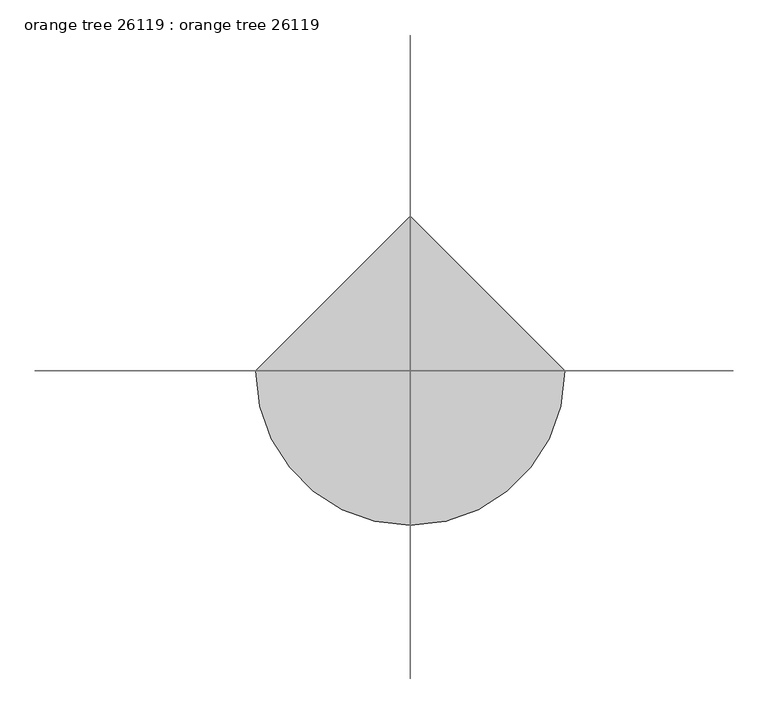
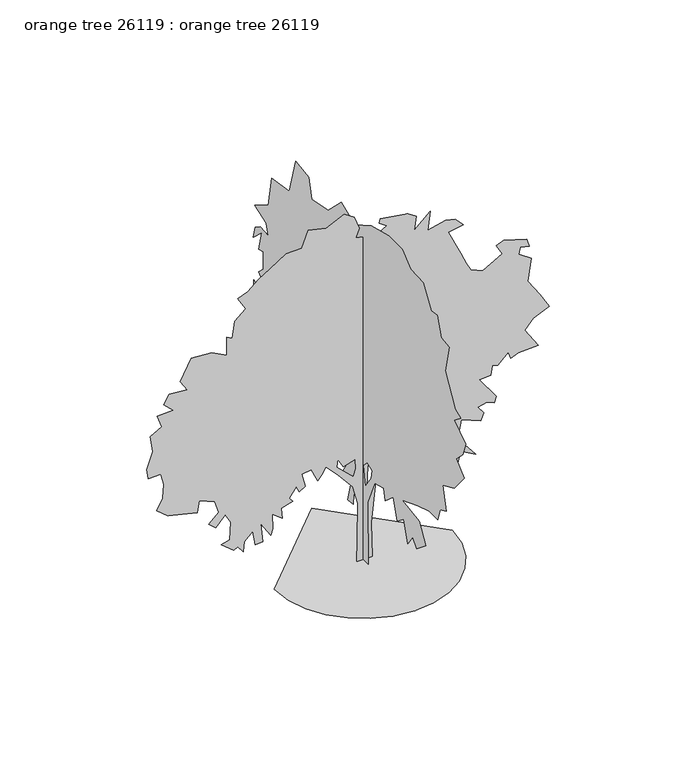
"""IFC4 building model written with IfcOpenShell, lengths in millimetres: proxy geometry, orange tree 26119 : orange tree 26119."""

import ifcopenshell
import ifcopenshell.guid

model = None  # the IFC model being written
_history = None  # IfcOwnerHistory: only IFC2X3 demands one
_inside = {}  # id of a spatial element -> (the spatial element, [elements in it])
_under = {}  # id of a project, library or spatial element -> (it, [spatial elements below it])
_declared = {}  # id of a project -> (the project, [libraries it declares])
_typed = {}  # id of a type object -> (the type object, [elements of that type])
_made_of = {}  # id of a material, layer set ... -> (it, [elements and type objects made of it])


def new_model(schema):
    """Start an empty IFC model of exactly this schema.

    Asked for "IFC4X3", IfcOpenShell would pick the latest addendum, in which some entities
    have other attributes; the version numbers below select the first issue.
    IFC2X3 requires an IfcOwnerHistory on every rooted entity: one is made here for all.
    """
    global model, _history
    if schema == "IFC4X3":
        model = ifcopenshell.file(schema_version=(4, 3, 0, 0))
    else:
        model = ifcopenshell.file(schema=schema)
    _inside.clear()
    _under.clear()
    _declared.clear()
    _typed.clear()
    _made_of.clear()
    _history = None
    if model.schema == "IFC2X3":
        org = make("IfcOrganization", Name="unknown")
        user = make(
            "IfcPersonAndOrganization",
            ThePerson=make("IfcPerson", FamilyName="unknown"),
            TheOrganization=org,
        )
        app = make(
            "IfcApplication",
            ApplicationDeveloper=org,
            Version="unknown",
            ApplicationFullName="unknown",
            ApplicationIdentifier="unknown",
        )
        _history = make(
            "IfcOwnerHistory",
            OwningUser=user,
            OwningApplication=app,
            ChangeAction="ADDED",
            CreationDate=0,
        )
    return model


def make(cls, **values):
    """One entity of the class cls with the attributes given. An attribute that is None is left unset."""
    return model.create_entity(
        cls, **{name: value for name, value in values.items() if value is not None}
    )


def rooted(cls, **values):
    """An entity with a GlobalId (a new one), such as an element, a storey or a relation."""
    return make(cls, GlobalId=ifcopenshell.guid.new(), OwnerHistory=_history, **values)


def si_unit(unit_type, name, prefix=None):
    """IfcSIUnit, for example si_unit("LENGTHUNIT", "METRE", prefix="MILLI")."""
    return make("IfcSIUnit", UnitType=unit_type, Prefix=prefix, Name=name)


def assignment(units):
    """IfcUnitAssignment: the units of a project."""
    return None if units is None else make("IfcUnitAssignment", Units=units)


def point(xyz):
    """IfcCartesianPoint."""
    return None if xyz is None else make("IfcCartesianPoint", Coordinates=xyz)


def direction(xyz):
    """IfcDirection."""
    return None if xyz is None else make("IfcDirection", DirectionRatios=xyz)


def frame(location, z_axis=None, x_axis=None):
    """IfcAxis2Placement3D, a coordinate frame: its origin and axes. An axis left out is left unset."""
    return make(
        "IfcAxis2Placement3D",
        Location=point(location),
        Axis=direction(z_axis),
        RefDirection=direction(x_axis),
    )


def origin():
    """The frame at (0, 0, 0) with its axes left unset."""
    return frame((0.0, 0.0, 0.0))


def place(relative_to, where):
    """IfcLocalPlacement: puts the frame where relative to a parent placement (None: the world)."""
    return make(
        "IfcLocalPlacement", PlacementRelTo=relative_to, RelativePlacement=where
    )


def context(
    kind, dimensions, precision=None, world=None, true_north=None, identifier=None
):
    """IfcGeometricRepresentationContext, for example the 3D "Model" context."""
    return make(
        "IfcGeometricRepresentationContext",
        ContextIdentifier=identifier,
        ContextType=kind,
        CoordinateSpaceDimension=dimensions,
        Precision=precision,
        WorldCoordinateSystem=world,
        TrueNorth=true_north,
    )


def project(units=None, contexts=None):
    """IfcProject with its units and contexts."""
    return rooted(
        "IfcProject",
        Name="project",
        RepresentationContexts=contexts,
        UnitsInContext=assignment(units),
    )


def spatial(cls, under=None, at=None, **own):
    """A site, building, storey or space (cls), placed at a placement, below another one or the project."""
    s = rooted(cls, ObjectPlacement=at, **own)
    if under is not None:
        _under.setdefault(under.id(), (under, []))[1].append(s)
    return s


def point_list(points):
    """IfcCartesianPointList2D or 3D."""
    cls = (
        "IfcCartesianPointList2D" if len(points[0]) == 2 else "IfcCartesianPointList3D"
    )
    return make(cls, CoordList=points)


def triangles(points, corners, closed=None, point_numbers=None):
    """IfcTriangulatedFaceSet: each triangle names its three corners, points numbered from 1."""
    return make(
        "IfcTriangulatedFaceSet",
        Coordinates=point_list(points),
        Closed=closed,
        CoordIndex=corners,
        PnIndex=point_numbers,
    )


def shape(context_of_items, identifier, shape_type, items):
    """IfcShapeRepresentation: the items that make up one representation, for example the "Body"."""
    return make(
        "IfcShapeRepresentation",
        ContextOfItems=context_of_items,
        RepresentationIdentifier=identifier,
        RepresentationType=shape_type,
        Items=items,
    )


def source(mapping_origin, context_of_items, identifier, shape_type, items):
    """IfcRepresentationMap: a shape defined once, which mapped items show again and again."""
    return make(
        "IfcRepresentationMap",
        MappingOrigin=mapping_origin,
        MappedRepresentation=shape(context_of_items, identifier, shape_type, items),
    )


def transform(
    local_origin,
    x_axis=None,
    y_axis=None,
    z_axis=None,
    scale=None,
    scale2=None,
    scale3=None,
    uniform=True,
):
    """IfcCartesianTransformationOperator3D, or its non-uniform kind. x_axis, y_axis, z_axis: its Axis1, 2, 3."""
    if uniform:
        return make(
            "IfcCartesianTransformationOperator3D",
            Axis1=direction(x_axis),
            Axis2=direction(y_axis),
            LocalOrigin=point(local_origin),
            Scale=scale,
            Axis3=direction(z_axis),
        )
    return make(
        "IfcCartesianTransformationOperator3DnonUniform",
        Axis1=direction(x_axis),
        Axis2=direction(y_axis),
        LocalOrigin=point(local_origin),
        Scale=scale,
        Axis3=direction(z_axis),
        Scale2=scale2,
        Scale3=scale3,
    )


def mapped(mapping_source, mapping_target):
    """IfcMappedItem: shows the shape of a source again, moved by a transform."""
    return make(
        "IfcMappedItem", MappingSource=mapping_source, MappingTarget=mapping_target
    )


def made_of(thing, what):
    """Note that an element or type object is made of a material, layer set ...; save() writes the relation."""
    if what is not None:
        _made_of.setdefault(what.id(), (what, []))[1].append(thing)
    return thing


def element(
    cls,
    number,
    at=None,
    inside=None,
    cuts=None,
    type_object=None,
    material=None,
    context=None,
    identifier="Body",
    shape_type=None,
    held_by="IfcProductDefinitionShape",
    body=None,
    shapes=None,
    **own,
):
    """One element of the class cls, such as IfcWall. Its Tag is "e" and its number.

    at: its placement. inside: the storey or other place that contains it. cuts: it is an
    opening in that element (IfcRelVoidsElement). A single representation is given by context,
    identifier, shape_type and body (its items); several are given by shapes. held_by: the class
    of the entity that holds the representations. save() writes the other relations.
    """
    e = rooted(cls, Tag="e%d" % number, ObjectPlacement=at, **own)
    if body is not None:
        shapes = [shape(context, identifier, shape_type, body)]
    if shapes is not None:
        e.Representation = make(held_by, Representations=shapes)
    if inside is not None:
        _inside.setdefault(inside.id(), (inside, []))[1].append(e)
    if cuts is not None:
        rooted(
            "IfcRelVoidsElement", RelatingBuildingElement=cuts, RelatedOpeningElement=e
        )
    if type_object is not None:
        _typed.setdefault(type_object.id(), (type_object, []))[1].append(e)
    return made_of(e, material)


def aggregate(whole, parts):
    """IfcRelAggregates: a whole, such as a stair, and the parts it consists of."""
    return rooted("IfcRelAggregates", RelatingObject=whole, RelatedObjects=parts)


def save(model, path):
    """Write the relations noted so far, then the file.

    IfcRelAggregates (storeys below a building ...), IfcRelContainedInSpatialStructure (elements
    in a storey), IfcRelDefinesByType, IfcRelAssociatesMaterial and IfcRelDeclares: one each for
    every whole, place, type object, material and project.
    """
    for whole, parts in _under.values():
        aggregate(whole, parts)
    for where, things in _inside.values():
        rooted(
            "IfcRelContainedInSpatialStructure",
            RelatedElements=things,
            RelatingStructure=where,
        )
    for kind, things in _typed.values():
        rooted("IfcRelDefinesByType", RelatedObjects=things, RelatingType=kind)
    for what, things in _made_of.values():
        rooted("IfcRelAssociatesMaterial", RelatedObjects=things, RelatingMaterial=what)
    for by, libraries in _declared.values():
        rooted("IfcRelDeclares", RelatingContext=by, RelatedDefinitions=libraries)
    model.write(path)


def orange_tree_26119_orange_tree_26119_d7a228f7(model_context):
    return source(origin(), model_context, "Body", "Tessellation", [
        triangles([(-803.9534712, 0.0, 6.05e-05), (-782.6987366, -184.2127929, 6.05e-05), (-722.1679836, -353.3826814, 6.05e-05), (-627.2075008, -502.663613, 6.05e-05), (-502.663613, -627.2075008, 6.05e-05), (-353.3826814, -722.1679836, 6.05e-05), (-184.2125386, -782.6987366, 6.05e-05), (3.51e-05, -803.9534712, 6.05e-05), (184.2127929, -782.6987366, 6.05e-05), (353.3826814, -722.1679836, 6.05e-05), (502.663613, -627.2075008, 6.05e-05), (627.2075008, -502.663613, 6.05e-05), (722.1679836, -353.3826814, 6.05e-05), (782.6987366, -184.2125386, 6.05e-05), (803.9534712, 7.03e-05, 6.05e-05), (-0.0001054, 803.9534712, 6.05e-05), (-4.73e-05, -77.0963933, 4.81e-05), (-2.95e-05, -72.7562921, 588.9525321), (-2.7e-05, -181.2628458, 836.3460434), (-3.2e-05, -320.1518609, 875.4087753), (-3.63e-05, -346.1919502, 771.2433311), (-3.87e-05, -472.0617019, 879.7495714), (-4.71e-05, -532.8235817, 688.7770712), (-4.92e-05, -632.6507006, 766.9024624), (-5.78e-05, -693.4151602, 571.5916368), (-5.81e-05, -775.878804, 684.4387459), (-6.3e-05, -832.3023949, 606.3134274), (-6.59e-05, -979.8713671, 727.8398031), (-5.62e-05, -875.7059229, 897.110503), (-4.32e-05, -610.9489002, 936.1731623), (-5.12e-05, -849.6633265, 1027.3185436), (-5.75e-05, -1031.9540892, 1088.0830032), (-6.35e-05, -1166.5029985, 1088.0830032), (-6.17e-05, -1201.224789, 1200.9301849), (-6.47e-05, -1296.7111118, 1244.3311695), (-5.59e-05, -1244.6283897, 1461.3462662), (-6.14e-05, -1422.5782837, 1543.8099827), (-6.28e-05, -1578.8289207, 1730.4416142), (-5.38e-05, -1452.9591328, 1843.2887959), (-5.55e-05, -1552.7863243, 1938.7749733), (-5.37e-05, -1600.5281776, 2068.9830139), (-4.21e-05, -1418.2374149, 2186.1685936), (-4.43e-05, -1526.7437279, 2272.9730335), (-3.95e-05, -1439.9391426, 2303.3564987), (-2.42e-05, -1279.3501076, 2576.8055054), (-1.94e-05, -1344.4529652, 2837.2061806), (-1.34e-05, -1218.5857206, 2850.2364899), (-5.3e-06, -1157.821261, 3028.1889999), (-1.5e-06, -1062.3375544, 3015.1586906), (9.7e-06, -940.8087078, 3206.14151), (1.89e-05, -741.1570135, 3214.8028999), (2.81e-05, -606.6080678, 3323.3116837), (3.75e-05, -398.2746723, 3327.6550232), (4.77e-05, -124.839264, 3258.2115875), (5.48e-05, 135.5766083, 3106.2941162), (6.66e-05, 339.5701524, 3197.4545403), (6.98e-05, 543.560172, 2997.8106216), (7.98e-05, 799.6379642, 2950.0585945), (8.73e-05, 847.3798176, 3128.0111046), (9.73e-05, 1051.3723806, 3158.3894829), (9.14e-05, 1151.1994995, 2811.1714325), (0.0001025, 1428.9739689, 2767.7627449), (9.64e-05, 1485.3975597, 2476.9656693), (0.0001018, 1689.3900501, 2351.0983521), (9.21e-05, 1515.7810249, 2285.9956398), (8.75e-05, 1481.0591618, 2186.1685936), (9.36e-05, 1606.926479, 2199.1910545), (9.54e-05, 1685.0517975, 2142.767609), (9.34e-05, 1715.4327919, 2029.9204273), (9.11e-05, 1580.8837372, 2155.7875992), (8.77e-05, 1632.9664593, 1964.815099), (8.51e-05, 1559.1820095, 1986.5168266), (8.02e-05, 1563.5228783, 1817.2460541), (8.14e-05, 1632.9664593, 1752.1433418), (7.34e-05, 1524.4602917, 1647.9754269), (7.38e-05, 1585.2246059, 1569.8525791), (8.13e-05, 1711.0919231, 1630.6144226), (7.79e-05, 1719.7736607, 1504.7472507), (7.16e-05, 1645.9890656, 1404.9226753), (7.48e-05, 1728.4527821, 1387.5618164), (7.27e-05, 1745.813641, 1292.0754936), (6.99e-05, 1650.3299343, 1339.817347), (6.11e-05, 1459.3574341, 1331.1382256), (6.23e-05, 1628.6282066, 1118.463925), (5.81e-05, 1520.1218937, 1140.1657253), (5.99e-05, 1611.2673477, 1062.0404068), (5.99e-05, 1698.0717876, 931.8322935), (5.77e-05, 1637.307328, 949.1932251), (5.11e-05, 1576.5454845, 818.9851845), (5.33e-05, 1572.2046158, 901.4513718), (4.88e-05, 1450.6756966, 931.8322935), (4.52e-05, 1402.9338432, 884.0904402), (4.47e-05, 1281.4075401, 1049.020344), (3.92e-05, 1264.0440651, 888.4313089), (3.71e-05, 1194.6004841, 923.1530994), (3.64e-05, 1116.4751656, 1018.6394222), (2.99e-05, 999.2896585, 975.2358215), (2.55e-05, 955.8861305, 892.7696342), (2.14e-05, 964.567868, 740.8623367), (1.6e-05, 873.4224867, 697.4588087), (1.6e-05, 916.8234713, 632.353553), (1.37e-05, 938.5251989, 523.8472401), (7.6e-06, 743.2143734, 610.6542961), (6.3e-06, 656.4073174, 697.4588087), (2.2e-06, 608.665464, 632.353553), (5.3e-06, 578.2845423, 779.9225252), (9e-07, 521.8609514, 719.1606091), (-7e-07, 456.7556594, 762.5615936), (1.1e-06, 465.4373606, 810.3059904), (-2e-06, 395.9937432, 810.3059904), (-7.3e-06, 335.22932, 723.5014778), (-6e-06, 291.8257738, 832.0077181), (-1e-05, 257.1039651, 749.5415308), (-1.02e-05, 317.8683884, 649.7169554), (-1.72e-05, 122.5560549, 710.4788715), (-1.74e-05, 192.000181, 597.6317262), (-2.03e-05, 244.0831574, 424.0226646), (-2.39e-05, 157.2781179, 432.7018224), (-2.16e-05, 144.2573102, 528.1880725), (-2.27e-05, 92.1740885, 571.5916368), (-2.48e-05, 44.4312178, 571.5916368), (-3.04e-05, 40.0908669, 389.3008378), (-4.11e-05, 61.7923765, 5.22e-05), (-2.23e-05, -137.8603261, 927.4914248), (-2.41e-05, -124.8395184, 849.3686497), (-2.39e-05, -33.6941257, 719.1606091), (-1.71e-05, -3.3121102, 901.4513718), (-1.8e-05, -64.07584, 962.2158314), (58.7260893, 2.69e-05, 920.6994701), (38.9260215, 3.03e-05, 877.8014345), (32.3258294, 4.22e-05, 683.1001648), (45.5259593, 4.5e-05, 626.9992287), (78.5256484, 3.59e-05, 755.7010386), (104.9259083, 2.72e-05, 881.1008698), (-56.7740963, 8.68e-05, 0.0), (-53.4738754, 7.45e-05, 204.6001204), (-50.1739042, 5.35e-05, 554.4008984), (-93.0740155, 4.51e-05, 726.0008165), (-225.0743068, 4.16e-05, 881.1008698), (-337.2739989, 3.93e-05, 1003.2012657), (-363.6747857, 4.36e-05, 950.3996922), (-409.8748363, 4.89e-05, 894.3012995), (-465.9733017, 4.39e-05, 1019.7011307), (-551.7745325, 4.85e-05, 1006.500701), (-522.0743105, 5.46e-05, 881.1008698), (-574.8733043, 5.89e-05, 848.1012125), (-604.5735263, 5.67e-05, 907.4991131), (-667.2734419, 6.47e-05, 818.4009905), (-634.2737846, 6.56e-05, 778.799774), (-739.8743156, 7.2e-05, 749.099552), (-729.9733938, 7.77e-05, 646.8010723), (-819.0740599, 7.74e-05, 716.0998947), (-815.7746246, 8.54e-05, 580.7991417), (-832.2744169, 8.94e-05, 524.7006763), (-924.6745909, 8.52e-05, 663.3008646), (-904.8752907, 9.48e-05, 488.3989677), (-970.8746778, 9.8e-05, 481.8000609), (-997.2754646, 9.11e-05, 617.1008503), (-1069.8737223, 9.86e-05, 544.4999765), (-1079.7746441, 0.0001046, 452.0998389), (-1129.2741663, 0.0001028, 518.0991898), (-1165.5758749, 0.0001058, 495.0004543), (-1281.0748569, 0.0001051, 590.7000635), (-1201.8750401, 0.0001005, 610.4993637), (-1195.2735535, 9.05e-05, 772.2009035), (-1241.4736404, 8.73e-05, 861.2990261), (-1327.2749439, 9.65e-05, 768.9013956), (-1389.9747505, 9.61e-05, 821.7004257), (-1300.8740845, 8.71e-05, 907.4991131), (-1337.1733223, 8.2e-05, 1019.7011307), (-1479.0755619, 8.49e-05, 1075.799596), (-1495.5752815, 9.19e-05, 970.2015358), (-1759.5754463, 9.97e-05, 1032.9014877), (-1858.5744907, 9.91e-05, 1115.4007399), (-1805.7755333, 9.07e-05, 1217.6992195), (-1799.1740467, 8.25e-05, 1349.70061), (-1825.5747608, 7.76e-05, 1451.999017), (-1937.7743076, 8.27e-05, 1448.6996544), (-1950.9746647, 7.78e-05, 1541.0998283), (-1894.8735832, 6.63e-05, 1692.9004463), (-1917.9749348, 5.84e-05, 1841.4015564), (-1815.6739117, 5.04e-05, 1900.7993843), (-1855.2749828, 4.52e-05, 2016.3009098), (-1713.3753593, 3.86e-05, 2022.8997803), (-1799.1740467, 3.75e-05, 2105.4015759), (-1746.3750893, 3.05e-05, 2184.6013927), (-1584.6734768, 2.4e-05, 2174.7003983), (-1650.6754074, 2.1e-05, 2273.6994427), (-1548.3743843, 5.5e-06, 2458.4999359), (-1366.8735443, -1.9e-06, 2448.6014122), (-1228.2732834, -3.6e-06, 2376.0006111), (-1228.2732834, -1.38e-05, 2547.5953697), (-1178.7737612, -1.44e-05, 2521.1995972), (-1158.974461, -2.45e-05, 2676.2973976), (-1056.6733652, -3.39e-05, 2758.7964317), (-1132.5736742, -3.79e-05, 2880.8942116), (-1040.1735003, -4.41e-05, 2917.1908333), (-941.1744558, -5.33e-05, 2999.6901581), (-835.5739248, -6.19e-05, 3065.7047333), (-693.6742287, -7.36e-05, 3158.1101395), (-555.0740041, -7.98e-05, 3161.4119728), (-495.6735237, -9.13e-05, 3309.9005836), (-333.9745637, -9.62e-05, 3273.6039619), (-172.2735144, -0.000108, 3352.8011627), (-79.8736311, -0.0001083, 3290.0884209), (-36.9737765, -0.0001029, 3167.990641), (-66.673751, -9.71e-05, 3092.0952736), (114.8263214, -0.0001024, 3049.1946945), (213.8264105, -0.0001101, 3105.303479), (144.5262982, -0.00011, 3154.8080154), (154.426457, -0.0001128, 3194.4067612), (401.9271747, -0.0001213, 3154.8080154), (477.8274837, -0.0001215, 3102.001355), (461.327655, -0.0001133, 2976.6014511), (606.5267864, -0.0001275, 3108.6053123), (580.126036, -0.0001159, 2933.700872), (745.1270473, -0.0001255, 2973.2996178), (827.6262268, -0.0001279, 2953.5130348), (900.2271006, -0.0001263, 2874.2902542), (768.2257828, -0.000119, 2847.8997139), (877.125749, -0.0001096, 2610.3081116), (929.9273226, -0.0001052, 2498.1010071), (969.525923, -0.0001024, 2422.2006981), (1078.4258892, -0.0001042, 2372.7011032), (1253.3278587, -0.000118, 2474.9995102), (1197.2268499, -0.0001212, 2570.7093658), (1266.525745, -0.000126, 2600.4020302), (1474.4272991, -0.0001312, 2534.4002449), (1497.5260345, -0.0001279, 2461.8017693), (1415.0268551, -0.0001252, 2478.3016342), (1401.826498, -0.0001211, 2418.9011902), (1514.0258995, -0.0001213, 2339.7013733), (1481.0261696, -0.0001075, 2131.7998192), (1593.2257164, -0.0001027, 1970.1008228), (1679.0268745, -9.78e-05, 1824.9016914), (1530.5257645, -8.76e-05, 1762.1992687), (1457.9274342, -7.91e-05, 1673.1010735), (1576.7258514, -7.35e-05, 1491.6002335), (1398.5269901, -6.51e-05, 1481.6993843), (1329.2255516, -6.03e-05, 1451.999017), (1309.4263241, -6.32e-05, 1514.701585), (1213.7267149, -5.39e-05, 1428.9002815), (1160.9276848, -5.24e-05, 1442.1006386), (1151.026763, -4.66e-05, 1352.9999725), (1045.426232, -4.18e-05, 1349.70061), (1197.2268499, -3.59e-05, 1138.4994753), (1180.726985, -3.16e-05, 1079.1015747), (1114.7275978, -3.05e-05, 1108.7992533), (1032.2258749, -2.57e-05, 1088.9999531), (1085.0273758, -2.39e-05, 1019.7011307), (1058.626589, -1.86e-05, 950.3996922), (883.7272356, -1.53e-05, 1023.0005659), (854.0270136, -3.8e-06, 851.4006477), (1012.4265747, 1.3e-06, 650.1005075), (877.125749, 2.7e-06, 726.0008165), (830.9257347, 1.63e-05, 531.2995831), (801.2255127, 1.04e-05, 653.3999428), (745.1270473, 8.7e-06, 722.7013813), (642.8259516, 1.59e-05, 676.5012943), (586.7274862, 2.47e-05, 570.900727), (487.725862, 2.15e-05, 696.3005945), (392.0262528, 1.76e-05, 831.6013475), (349.1256374, 2.48e-05, 742.5006815), (316.1259439, 1.76e-05, 887.6998129), (187.4264049, 2.7e-05, 824.999861), (114.8263214, 3.72e-05, 706.1989729), (71.9262193, 6.15e-05, 329.999443), (81.8261282, 8.08e-05, 0.0001067), (-178.8742198, 3.57e-05, 947.1002569), (-228.3742689, 3.25e-05, 1036.200923), (-238.2741733, 3.73e-05, 963.6001219), (-89.7740443, 3.95e-05, 818.4009905), (-66.6740053, 3.43e-05, 887.6998129), (-73.2739431, 2.91e-05, 980.0999868)], [[15, 16, 1], [14, 15, 1], [14, 1, 2], [13, 14, 2], [13, 2, 3], [13, 3, 4], [12, 13, 4], [11, 12, 4], [11, 4, 5], [11, 5, 6], [11, 6, 7], [11, 7, 8], [11, 8, 9], [11, 9, 10], [126, 17, 18], [88, 89, 90], [68, 69, 70], [67, 68, 70], [83, 84, 85], [86, 87, 88], [126, 18, 19], [125, 126, 19], [113, 114, 115], [104, 105, 106], [63, 64, 65], [80, 81, 82], [79, 80, 82], [66, 67, 70], [24, 25, 26], [101, 102, 103], [110, 111, 112], [42, 43, 44], [70, 71, 72], [20, 21, 22], [100, 101, 103], [116, 117, 118], [116, 118, 119], [76, 77, 78], [22, 23, 24], [93, 94, 95], [93, 95, 96], [76, 78, 79], [91, 92, 93], [45, 46, 47], [116, 119, 120], [115, 116, 120], [26, 27, 28], [26, 28, 29], [26, 29, 30], [24, 26, 30], [22, 24, 30], [123, 17, 126], [122, 123, 126], [121, 122, 126], [73, 74, 75], [79, 82, 83], [76, 79, 83], [37, 38, 39], [124, 125, 19], [59, 60, 61], [58, 59, 61], [106, 107, 108], [106, 108, 109], [66, 70, 72], [124, 19, 20], [34, 35, 36], [47, 48, 49], [100, 103, 104], [115, 120, 121], [115, 121, 126], [115, 126, 127], [40, 41, 42], [39, 40, 42], [32, 33, 34], [113, 115, 127], [112, 113, 127], [61, 62, 63], [55, 56, 57], [98, 99, 100], [98, 100, 104], [98, 104, 106], [86, 88, 90], [86, 90, 91], [85, 86, 91], [85, 91, 93], [83, 85, 93], [75, 76, 83], [36, 37, 39], [49, 50, 51], [83, 93, 96], [32, 34, 36], [97, 98, 106], [31, 32, 36], [42, 44, 45], [97, 106, 109], [51, 52, 53], [75, 83, 96], [75, 96, 97], [61, 63, 65], [61, 65, 66], [58, 61, 66], [57, 58, 66], [75, 97, 109], [73, 75, 109], [72, 73, 109], [66, 72, 109], [57, 66, 109], [57, 109, 110], [57, 110, 112], [57, 112, 127], [57, 127, 128], [55, 57, 128], [54, 55, 128], [53, 54, 128], [51, 53, 128], [49, 51, 128], [47, 49, 128], [45, 47, 128], [42, 45, 128], [39, 42, 128], [36, 39, 128], [31, 36, 128], [30, 31, 128], [30, 128, 124], [30, 124, 20], [30, 20, 22], [135, 130, 131], [130, 135, 136], [130, 136, 137], [135, 131, 132], [253, 254, 255], [255, 256, 257], [130, 137, 138], [272, 129, 130], [272, 130, 138], [129, 272, 273], [262, 263, 264], [214, 215, 216], [272, 138, 139], [271, 272, 139], [271, 139, 140], [159, 160, 161], [150, 151, 152], [153, 154, 155], [152, 153, 155], [162, 163, 164], [218, 219, 220], [237, 238, 239], [228, 229, 230], [227, 228, 230], [191, 192, 193], [141, 142, 143], [148, 149, 150], [259, 260, 261], [182, 183, 184], [217, 218, 220], [161, 162, 164], [270, 271, 140], [129, 273, 274], [195, 196, 197], [268, 135, 132], [267, 268, 132], [266, 267, 132], [266, 132, 133], [265, 266, 133], [265, 133, 134], [246, 247, 248], [245, 246, 248], [234, 235, 236], [140, 141, 143], [225, 226, 227], [225, 227, 230], [225, 230, 231], [167, 168, 169], [166, 167, 169], [239, 240, 241], [145, 146, 147], [144, 145, 147], [255, 257, 258], [253, 255, 258], [171, 172, 173], [237, 239, 241], [216, 217, 220], [245, 248, 249], [250, 251, 252], [249, 250, 252], [155, 156, 157], [155, 157, 158], [210, 211, 212], [209, 210, 212], [177, 178, 179], [243, 244, 245], [201, 202, 203], [184, 185, 186], [184, 186, 187], [274, 269, 270], [173, 174, 175], [171, 173, 175], [159, 161, 164], [177, 179, 180], [158, 159, 164], [158, 164, 165], [155, 158, 165], [171, 175, 176], [180, 181, 182], [188, 189, 190], [187, 188, 190], [187, 190, 191], [231, 232, 233], [245, 249, 252], [212, 213, 214], [209, 212, 214], [203, 204, 205], [203, 205, 206], [203, 206, 207], [201, 203, 207], [264, 265, 134], [208, 209, 214], [241, 242, 243], [225, 231, 233], [224, 225, 233], [233, 234, 236], [224, 233, 236], [224, 236, 237], [224, 237, 241], [224, 241, 243], [223, 224, 243], [223, 243, 245], [152, 155, 165], [152, 165, 166], [259, 261, 262], [258, 259, 262], [253, 258, 262], [252, 253, 262], [252, 262, 264], [245, 252, 264], [223, 245, 264], [223, 264, 134], [223, 134, 129], [223, 129, 274], [223, 274, 270], [222, 223, 270], [221, 222, 270], [220, 221, 270], [216, 220, 270], [214, 216, 270], [208, 214, 270], [207, 208, 270], [201, 207, 270], [200, 201, 270], [199, 200, 270], [198, 199, 270], [197, 198, 270], [195, 197, 270], [194, 195, 270], [193, 194, 270], [191, 193, 270], [191, 270, 140], [191, 140, 143], [191, 143, 144], [187, 191, 144], [184, 187, 144], [182, 184, 144], [180, 182, 144], [177, 180, 144], [176, 177, 144], [171, 176, 144], [170, 171, 144], [170, 144, 147], [169, 170, 147], [166, 169, 147], [152, 166, 147], [152, 147, 148], [152, 148, 150]], closed=False),
    ])


if __name__ == "__main__":
    model = new_model("IFC4")
    model_context = context("Model", 3, world=origin())
    ifc_project = project(units=[si_unit("LENGTHUNIT", "METRE", prefix="MILLI")], contexts=[model_context])
    site = spatial("IfcSite", under=ifc_project)
    building = spatial("IfcBuilding", under=site)
    placement = place(None, origin())
    orange_tree_26119_orange_tree_26119_shape = orange_tree_26119_orange_tree_26119_d7a228f7(model_context)
    element("IfcBuildingElementProxy", 1, Name="orange tree 26119 : orange tree 26119", ObjectType="orange tree 26119 : orange tree 26119", at=placement, inside=building, context=model_context, shape_type="MappedRepresentation", body=[
        mapped(orange_tree_26119_orange_tree_26119_shape, transform((0.0, 0.0, 0.0), x_axis=(1.0, 0.0, 0.0), y_axis=(0.0, 1.0, 0.0), z_axis=(0.0, 0.0, 1.0))),
    ])
    save(model, "model.ifc")

# Revit data of these elements
# Type "orange tree 26119 : orange tree 26119"
#   built-in parameter 1005195 = "RPC-16-FVGW-4XXX-7J75-W000-ST1L-LVER-AU"
#   Height = 0
